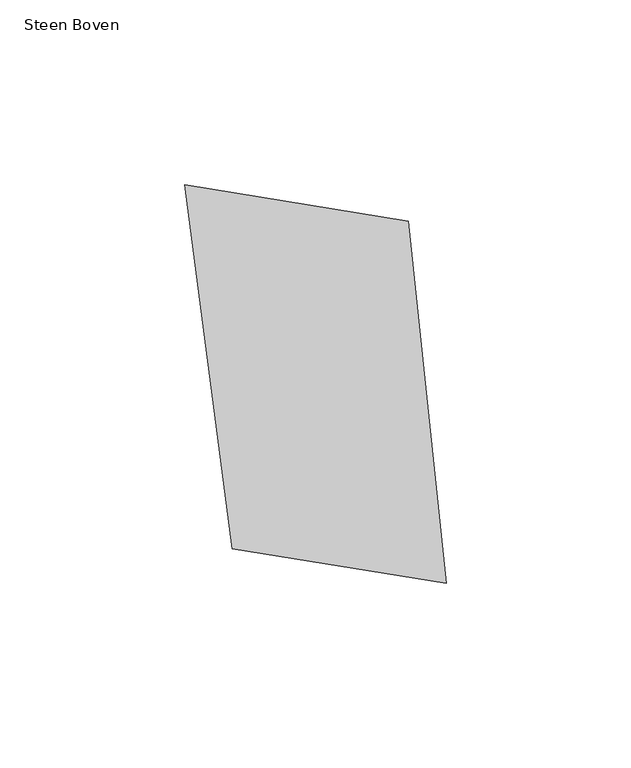
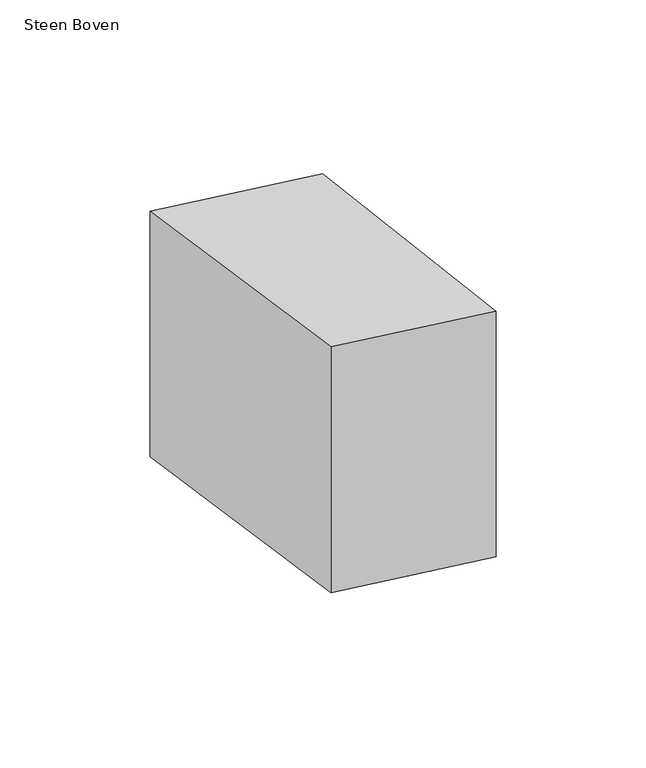
"""IFC4 building model written with IfcOpenShell, lengths in millimetres: proxy geometry, 00_GMA_steen_versie_4 : Steen Boven."""

from ifc_helpers import new_model, si_unit, origin, origin_with_axes, place, context, project, spatial, polyline, outline, extrude, source, transform, mapped, element, save


def steen_boven_18b6fb54(model_context):
    return source(origin(), model_context, "Body", "SweptSolid", [
        extrude(outline(polyline([(95.2647769, 120.9322109), (105.4545825, 22.8392806), (47.5152768, 32.2489504), (34.63584, 130.8115532), (95.2647769, 120.9322109)])), origin_with_axes(), (0.0, 0.0, 1.0), 100.0),
    ])


if __name__ == "__main__":
    model = new_model("IFC4")
    model_context = context("Model", 3, world=origin())
    ifc_project = project(units=[si_unit("LENGTHUNIT", "METRE", prefix="MILLI")], contexts=[model_context])
    site = spatial("IfcSite", under=ifc_project)
    building = spatial("IfcBuilding", under=site)
    placement = place(None, origin())
    steen_boven_shape = steen_boven_18b6fb54(model_context)
    element("IfcBuildingElementProxy", 1, Name="00_GMA_steen_versie_4 : Steen Boven", ObjectType="00_GMA_steen_versie_4 : Steen Boven", at=placement, inside=building, context=model_context, shape_type="MappedRepresentation", body=[
        mapped(steen_boven_shape, transform((0.0, 0.0, 0.0), x_axis=(1.0, 0.0, 0.0), y_axis=(0.0, 1.0, 0.0), z_axis=(0.0, 0.0, 1.0))),
    ])
    save(model, "model.ifc")

# Revit data of these elements
# Type "00_GMA_steen_versie_4 : Steen Boven"
#   StootVoegHalfBoven [instance default] = 5 mm
#   StootVoegHalf [instance default] = 5 mm
#   StootVoegBreedteOnder = 10 mm
#   StootVoegBreedteBoven = 10 mm
#   Steendikte = 100 mm
#   LintVoegOnderHalf = 5 mm
#   LintVoegOnder = 10 mm
#   LintVoegBovenHalf = 0 mm
#   LintVoegBoven = 0 mm
#   materiaal = none
#   MateriaalVoeg = none
#   Default Elevation = 0
